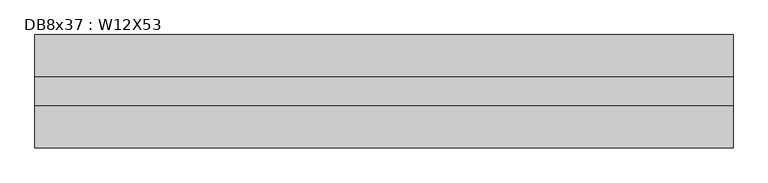
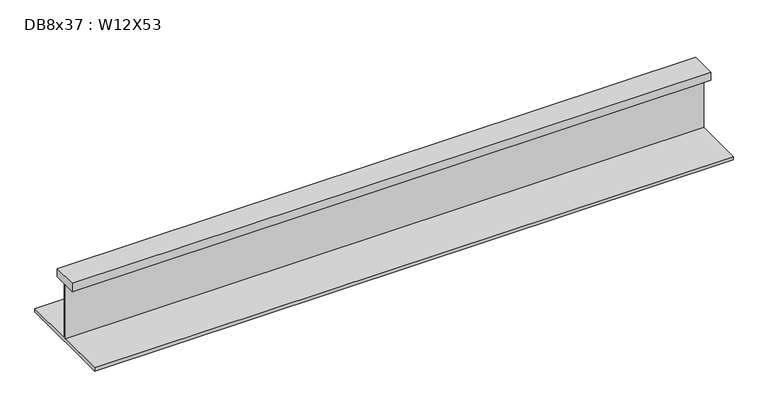
"""IFC4 building model written with IfcOpenShell, lengths in millimetres: beam geometry, DB8x37 : W12X53."""

from ifc_helpers import new_model, si_unit, frame, origin, place, context, project, spatial, polyline, outline, extrude, source, transform, mapped, element, save


def db8x37_w12x53_d2084d4f(model_context):
    return source(origin(), model_context, "Body", "SweptSolid", [
        extrude(outline(polyline([(38.1, 145.415), (38.1, 120.015), (2.921, 120.015), (2.921, -48.4505), (152.4, -48.4505), (152.4, -58.1025), (-152.4, -58.1025), (-152.4, -48.4505), (-2.921, -48.4505), (-2.921, 120.015), (-38.1, 120.015), (-38.1, 145.415), (38.1, 145.415)])), frame((-901.7, 0.0, 0.0), z_axis=(1.0, 0.0, 0.0), x_axis=(0.0, 1.0, 0.0)), (0.0, 0.0, 1.0), 1879.552375),
    ])


if __name__ == "__main__":
    model = new_model("IFC4")
    model_context = context("Model", 3, world=origin())
    ifc_project = project(units=[si_unit("LENGTHUNIT", "METRE", prefix="MILLI")], contexts=[model_context])
    site = spatial("IfcSite", under=ifc_project)
    building = spatial("IfcBuilding", under=site)
    placement = place(None, origin())
    db8x37_w12x53_shape = db8x37_w12x53_d2084d4f(model_context)
    element("IfcBeam", 1, ObjectType="DB8x37 : W12X53", at=placement, inside=building, context=model_context, shape_type="MappedRepresentation", body=[
        mapped(db8x37_w12x53_shape, transform((0.0, 0.0, 0.0), x_axis=(1.0, 0.0, 0.0), y_axis=(0.0, 1.0, 0.0), z_axis=(0.0, 0.0, 1.0))),
    ])
    save(model, "model.ifc")

# Revit data of these elements
# Type "DB8x37 : W12X53"
#   Assembly Code = "B10"
#   W = 53
#   Length [instance default] = 5' - 0"
#   bf = 0' - 10"
#   d = 1' - 0.1"
#   k = 0' - 1 3/8"
#   k2 = 0' - 0.8"
#   tf = 0' - 0.575"
#   tw = 0' - 0.345"
#   A = 0.108333 SF
#   Structural Material [instance default] = Steel ASTM A992
# Element 1 (IfcBeam, "DB8x37 : W12X53")
#   Materials on its faces: "Steel ASTM A992"
# Materials
#   "Steel ASTM A992": class "Metal", colour RGB 199 199 199, transparency 0, Description = "Structural steel 50ksi", Cost = 0
